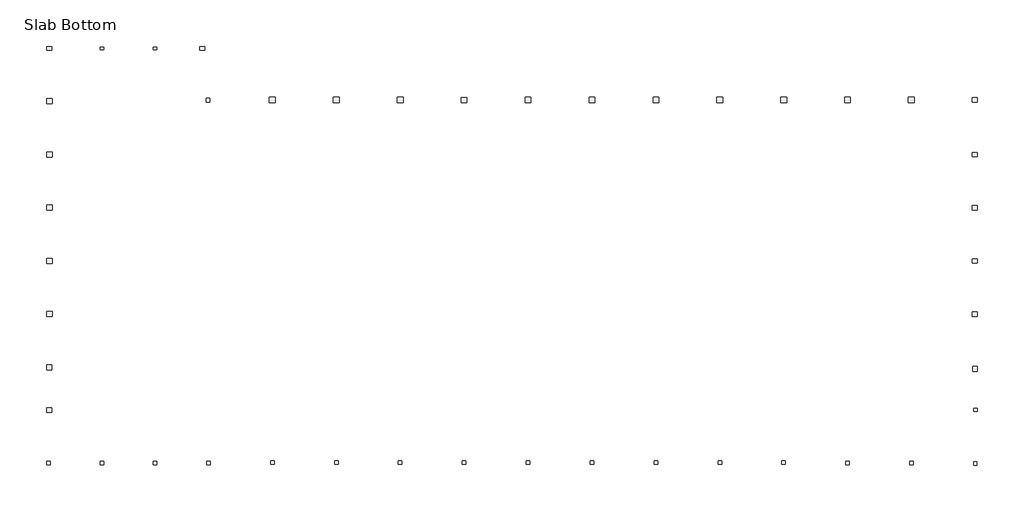
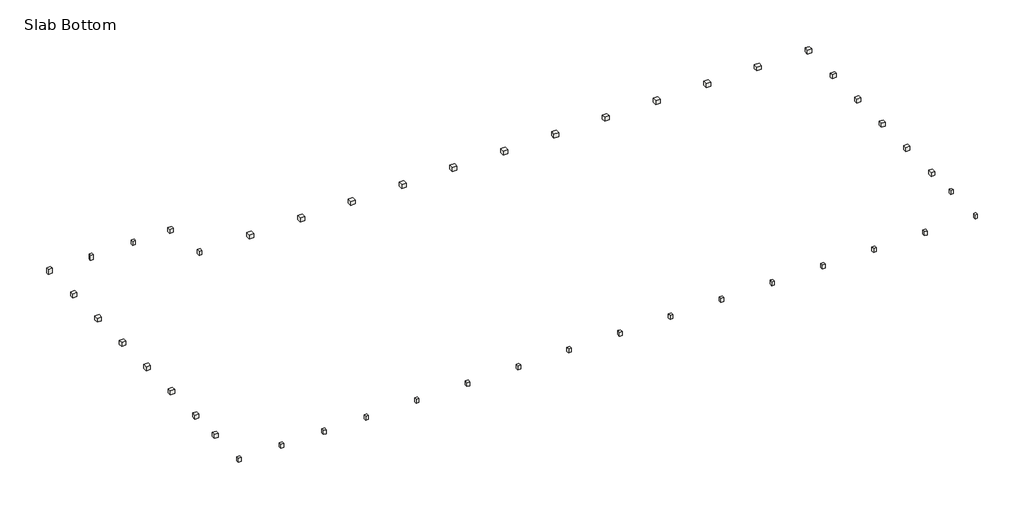
# One storey: 46 slabs.
"""IFC4 building model written with IfcOpenShell, lengths in millimetres."""

from ifc_helpers import new_model, si_unit, frame, origin, place, context, project, spatial, polyline, outline, extrude, faceted_brep, element, save

model = new_model("IFC4")

# Units and contexts
model_context = context("Model", 3, world=origin())
ifc_project = project(units=[si_unit("LENGTHUNIT", "METRE", prefix="MILLI")], contexts=[model_context])

# Site, building, storey
site = spatial("IfcSite", under=ifc_project)
building = spatial("IfcBuilding", under=site)
storey = spatial("IfcBuildingStorey", under=building, Name="Slab Bottom", Elevation=-152.4)

# Slabs
placement = place(None, origin())
element("IfcSlab", 1, ObjectType="Footing-Rectangular : P1", at=placement, inside=storey, context=model_context, shape_type="SweptSolid", body=[
    extrude(outline(polyline([(411310.2398264, -572441.1413841), (411665.8398264, -572441.1413841), (411665.8398264, -572745.9413841), (411310.2398264, -572745.9413841), (411310.2398264, -572441.1413841)])), frame((0.0, 0.0, -914.4), z_axis=(0.0, 0.0, 1.0), x_axis=(1.0, 0.0, 0.0)), (0.0, 0.0, 1.0), 609.6),
])
element("IfcSlab", 2, ObjectType="Footing-Rectangular : P11", at=placement, inside=storey, context=model_context, shape_type="SweptSolid", body=[
    extrude(outline(polyline([(411138.7898264, -549562.0913841), (411138.7898264, -549054.0913841), (411697.5898264, -549054.0913841), (411697.5898264, -549562.0913841), (411138.7898264, -549562.0913841)])), frame((0.0, 0.0, -914.4), z_axis=(0.0, 0.0, 1.0), x_axis=(1.0, 0.0, 0.0)), (0.0, 0.0, 1.0), 609.6),
])
element("IfcSlab", 3, ObjectType="Footing-Rectangular : P11A", at=placement, inside=storey, context=model_context, shape_type="SweptSolid", body=[
    extrude(outline(polyline([(411138.7898264, -561817.5913841), (411138.7898264, -561309.5913841), (411697.5898264, -561309.5913841), (411697.5898264, -561817.5913841), (411138.7898264, -561817.5913841)])), frame((0.0, 0.0, -914.4), z_axis=(0.0, 0.0, 1.0), x_axis=(1.0, 0.0, 0.0)), (0.0, 0.0, 1.0), 609.6),
])
element("IfcSlab", 4, ObjectType="Footing-Rectangular : P12", at=placement, inside=storey, context=model_context, shape_type="SweptSolid", body=[
    extrude(outline(polyline([(304649.2898264, -537331.9913841), (304649.2898264, -536773.1913841), (305258.8898264, -536773.1913841), (305258.8898264, -537331.9913841), (304649.2898264, -537331.9913841)])), frame((0.0, 0.0, -914.4), z_axis=(0.0, 0.0, 1.0), x_axis=(1.0, 0.0, 0.0)), (0.0, 0.0, 1.0), 609.6),
])
element("IfcSlab", 5, ObjectType="Footing-Rectangular : P12", at=placement, inside=storey, context=model_context, shape_type="SweptSolid", body=[
    extrude(outline(polyline([(304649.2898264, -543459.7413841), (304649.2898264, -542900.9413841), (305258.8898264, -542900.9413841), (305258.8898264, -543459.7413841), (304649.2898264, -543459.7413841)])), frame((0.0, 0.0, -914.4), z_axis=(0.0, 0.0, 1.0), x_axis=(1.0, 0.0, 0.0)), (0.0, 0.0, 1.0), 609.6),
])
element("IfcSlab", 6, ObjectType="Footing-Rectangular : P12", at=placement, inside=storey, context=model_context, shape_type="SweptSolid", body=[
    extrude(outline(polyline([(304649.2898264, -549587.4913841), (304649.2898264, -549028.6913841), (305258.8898264, -549028.6913841), (305258.8898264, -549587.4913841), (304649.2898264, -549587.4913841)])), frame((0.0, 0.0, -914.4), z_axis=(0.0, 0.0, 1.0), x_axis=(1.0, 0.0, 0.0)), (0.0, 0.0, 1.0), 609.6),
])
element("IfcSlab", 7, ObjectType="Footing-Rectangular : P12", at=placement, inside=storey, context=model_context, shape_type="SweptSolid", body=[
    extrude(outline(polyline([(304649.2898264, -555715.2413841), (304649.2898264, -555156.4413841), (305258.8898264, -555156.4413841), (305258.8898264, -555715.2413841), (304649.2898264, -555715.2413841)])), frame((0.0, 0.0, -914.4), z_axis=(0.0, 0.0, 1.0), x_axis=(1.0, 0.0, 0.0)), (0.0, 0.0, 1.0), 609.6),
])
element("IfcSlab", 8, ObjectType="Footing-Rectangular : P12", at=placement, inside=storey, context=model_context, shape_type="SweptSolid", body=[
    extrude(outline(polyline([(304649.2898264, -561842.9913841), (304649.2898264, -561284.1913841), (305258.8898264, -561284.1913841), (305258.8898264, -561842.9913841), (304649.2898264, -561842.9913841)])), frame((0.0, 0.0, -914.4), z_axis=(0.0, 0.0, 1.0), x_axis=(1.0, 0.0, 0.0)), (0.0, 0.0, 1.0), 609.6),
])
element("IfcSlab", 9, ObjectType="Footing-Rectangular : P12", at=placement, inside=storey, context=model_context, shape_type="SweptSolid", body=[
    extrude(outline(polyline([(304623.8898264, -567970.7413841), (304623.8898264, -567411.9413841), (305233.4898264, -567411.9413841), (305233.4898264, -567970.7413841), (304623.8898264, -567970.7413841)])), frame((0.0, 0.0, -914.4), z_axis=(0.0, 0.0, 1.0), x_axis=(1.0, 0.0, 0.0)), (0.0, 0.0, 1.0), 609.6),
])
element("IfcSlab", 10, ObjectType="Footing-Rectangular : P13", at=placement, inside=storey, context=model_context, shape_type="SweptSolid", body=[
    extrude(outline(polyline([(403777.974756, -536594.2315281), (404438.374756, -536594.2315281), (404438.374756, -537203.8315281), (403777.974756, -537203.8315281), (403777.974756, -536594.2315281)])), frame((0.0, 0.0, -914.4), z_axis=(0.0, 0.0, 1.0), x_axis=(1.0, 0.0, 0.0)), (0.0, 0.0, 1.0), 609.6),
])
element("IfcSlab", 11, ObjectType="Footing-Rectangular : P13", at=placement, inside=storey, context=model_context, shape_type="SweptSolid", body=[
    extrude(outline(polyline([(396451.2398264, -536601.7413358), (397111.6398264, -536601.7413358), (397111.6398264, -537211.3413358), (396451.2398264, -537211.3413358), (396451.2398264, -536601.7413358)])), frame((0.0, 0.0, -914.4), z_axis=(0.0, 0.0, 1.0), x_axis=(1.0, 0.0, 0.0)), (0.0, 0.0, 1.0), 609.6),
])
element("IfcSlab", 12, ObjectType="Footing-Rectangular : P13", at=placement, inside=storey, context=model_context, shape_type="SweptSolid", body=[
    extrude(outline(polyline([(389097.9398264, -536601.7413358), (389758.3398264, -536601.7413358), (389758.3398264, -537211.3413358), (389097.9398264, -537211.3413358), (389097.9398264, -536601.7413358)])), frame((0.0, 0.0, -914.4), z_axis=(0.0, 0.0, 1.0), x_axis=(1.0, 0.0, 0.0)), (0.0, 0.0, 1.0), 609.6),
])
element("IfcSlab", 13, ObjectType="Footing-Rectangular : P13", at=placement, inside=storey, context=model_context, shape_type="SweptSolid", body=[
    extrude(outline(polyline([(381744.6398264, -536601.7413358), (382405.0398264, -536601.7413358), (382405.0398264, -537211.3413358), (381744.6398264, -537211.3413358), (381744.6398264, -536601.7413358)])), frame((0.0, 0.0, -914.4), z_axis=(0.0, 0.0, 1.0), x_axis=(1.0, 0.0, 0.0)), (0.0, 0.0, 1.0), 609.6),
])
element("IfcSlab", 14, ObjectType="Footing-Rectangular : P13", at=placement, inside=storey, context=model_context, shape_type="SweptSolid", body=[
    extrude(outline(polyline([(374391.3398264, -536601.7413358), (375051.7398264, -536601.7413358), (375051.7398264, -537211.3413358), (374391.3398264, -537211.3413358), (374391.3398264, -536601.7413358)])), frame((0.0, 0.0, -914.4), z_axis=(0.0, 0.0, 1.0), x_axis=(1.0, 0.0, 0.0)), (0.0, 0.0, 1.0), 609.6),
])
element("IfcSlab", 15, ObjectType="Footing-Rectangular : P13", at=placement, inside=storey, context=model_context, shape_type="SweptSolid", body=[
    extrude(outline(polyline([(367038.0398264, -536601.7413358), (367698.4398264, -536601.7413358), (367698.4398264, -537211.3413358), (367038.0398264, -537211.3413358), (367038.0398264, -536601.7413358)])), frame((0.0, 0.0, -914.4), z_axis=(0.0, 0.0, 1.0), x_axis=(1.0, 0.0, 0.0)), (0.0, 0.0, 1.0), 609.6),
])
element("IfcSlab", 16, ObjectType="Footing-Rectangular : P13", at=placement, inside=storey, context=model_context, shape_type="SweptSolid", body=[
    extrude(outline(polyline([(359684.7398264, -536601.7413358), (360345.1398264, -536601.7413358), (360345.1398264, -537211.3413358), (359684.7398264, -537211.3413358), (359684.7398264, -536601.7413358)])), frame((0.0, 0.0, -914.4), z_axis=(0.0, 0.0, 1.0), x_axis=(1.0, 0.0, 0.0)), (0.0, 0.0, 1.0), 609.6),
])
element("IfcSlab", 17, ObjectType="Footing-Rectangular : P13", at=placement, inside=storey, context=model_context, shape_type="SweptSolid", body=[
    extrude(outline(polyline([(352331.4398264, -536614.4413358), (352991.8398264, -536614.4413358), (352991.8398264, -537224.0413358), (352331.4398264, -537224.0413358), (352331.4398264, -536614.4413358)])), frame((0.0, 0.0, -914.4), z_axis=(0.0, 0.0, 1.0), x_axis=(1.0, 0.0, 0.0)), (0.0, 0.0, 1.0), 609.6),
])
element("IfcSlab", 18, ObjectType="Footing-Rectangular : P13", at=placement, inside=storey, context=model_context, shape_type="SweptSolid", body=[
    extrude(outline(polyline([(344978.1398264, -536601.7413358), (345638.5398264, -536601.7413358), (345638.5398264, -537211.3413358), (344978.1398264, -537211.3413358), (344978.1398264, -536601.7413358)])), frame((0.0, 0.0, -914.4), z_axis=(0.0, 0.0, 1.0), x_axis=(1.0, 0.0, 0.0)), (0.0, 0.0, 1.0), 609.6),
])
element("IfcSlab", 19, ObjectType="Footing-Rectangular : P13", at=placement, inside=storey, context=model_context, shape_type="SweptSolid", body=[
    extrude(outline(polyline([(337624.8398264, -536601.7413358), (338285.2398264, -536601.7413358), (338285.2398264, -537211.3413358), (337624.8398264, -537211.3413358), (337624.8398264, -536601.7413358)])), frame((0.0, 0.0, -914.4), z_axis=(0.0, 0.0, 1.0), x_axis=(1.0, 0.0, 0.0)), (0.0, 0.0, 1.0), 609.6),
])
element("IfcSlab", 20, ObjectType="Footing-Rectangular : P13", at=placement, inside=storey, context=model_context, shape_type="SweptSolid", body=[
    extrude(outline(polyline([(330271.5398264, -536601.7413358), (330931.9398264, -536601.7413358), (330931.9398264, -537211.3413358), (330271.5398264, -537211.3413358), (330271.5398264, -536601.7413358)])), frame((0.0, 0.0, -914.4), z_axis=(0.0, 0.0, 1.0), x_axis=(1.0, 0.0, 0.0)), (0.0, 0.0, 1.0), 609.6),
])
element("IfcSlab", 21, ObjectType="Footing-Rectangular : P13A", at=placement, inside=storey, context=model_context, shape_type="SweptSolid", body=[
    extrude(outline(polyline([(411107.0397781, -536620.7913358), (411716.6397781, -536620.7913358), (411716.6397781, -537179.5913358), (411107.0397781, -537179.5913358), (411107.0397781, -536620.7913358)])), frame((0.0, 0.0, -914.4), z_axis=(0.0, 0.0, 1.0), x_axis=(1.0, 0.0, 0.0)), (0.0, 0.0, 1.0), 609.6),
])
element("IfcSlab", 22, ObjectType="Footing-Rectangular : P14", at=placement, inside=storey, context=model_context, shape_type="Brep", body=[
    faceted_brep([(304649.2898264, -572339.5413841, -304.8), (304649.2898264, -572847.5413841, -304.8), (305208.0898264, -572847.5413841, -304.8), (305208.0898264, -572810.8391729, -304.8), (305208.0898264, -572404.4391729, -304.8), (305208.0898264, -572339.5413841, -304.8), (304649.2898264, -572339.5413841, -914.4), (304649.2898264, -572847.5413841, -914.4), (305208.0898264, -572847.5413841, -914.4), (305208.0898264, -572339.5413841, -914.4)], [[[0, 1, 2, 3, 4, 5]], [[1, 0, 6, 7]], [[2, 1, 7, 8]], [[5, 4, 3, 2, 8, 9]], [[0, 5, 9, 6]], [[7, 6, 9, 8]]]),
])
element("IfcSlab", 23, ObjectType="Footing-Rectangular : P2", at=placement, inside=storey, context=model_context, shape_type="SweptSolid", body=[
    extrude(outline(polyline([(322797.5898264, -530747.0413841), (322797.5898264, -531153.4413841), (322238.7898264, -531153.4413841), (322238.7898264, -530747.0413841), (322797.5898264, -530747.0413841)])), frame((0.0, 0.0, -914.4), z_axis=(0.0, 0.0, 1.0), x_axis=(1.0, 0.0, 0.0)), (0.0, 0.0, 1.0), 609.6),
])
element("IfcSlab", 24, ObjectType="Footing-Rectangular : P3", at=placement, inside=storey, context=model_context, shape_type="SweptSolid", body=[
    extrude(outline(polyline([(411310.2398264, -578543.4913841), (411615.0398264, -578543.4913841), (411615.0398264, -578949.8913841), (411310.2398264, -578949.8913841), (411310.2398264, -578543.4913841)])), frame((0.0, 0.0, -914.4), z_axis=(0.0, 0.0, 1.0), x_axis=(1.0, 0.0, 0.0)), (0.0, 0.0, 1.0), 609.6),
])
element("IfcSlab", 25, ObjectType="Footing-Rectangular : P4", at=placement, inside=storey, context=model_context, shape_type="SweptSolid", body=[
    extrude(outline(polyline([(310789.7398264, -531108.9913841), (310789.7398264, -530804.1913841), (311196.1398264, -530804.1913841), (311196.1398264, -531108.9913841), (310789.7398264, -531108.9913841)])), frame((0.0, 0.0, -1066.8), z_axis=(0.0, 0.0, 1.0), x_axis=(1.0, 0.0, 0.0)), (0.0, 0.0, 1.0), 762.0),
])
element("IfcSlab", 26, ObjectType="Footing-Rectangular : P4", at=placement, inside=storey, context=model_context, shape_type="SweptSolid", body=[
    extrude(outline(polyline([(317323.8898264, -531108.9913841), (316917.4898264, -531108.9913841), (316917.4898264, -530804.1913841), (317323.8898264, -530804.1913841), (317323.8898264, -531108.9913841)])), frame((0.0, 0.0, -914.4), z_axis=(0.0, 0.0, 1.0), x_axis=(1.0, 0.0, 0.0)), (0.0, 0.0, 1.0), 609.6),
])
element("IfcSlab", 27, ObjectType="Footing-Rectangular : P5", at=placement, inside=storey, context=model_context, shape_type="SweptSolid", body=[
    extrude(outline(polyline([(311196.1398264, -578892.7413841), (310789.7398264, -578892.7413841), (310789.7398264, -578486.3413841), (311196.1398264, -578486.3413841), (311196.1398264, -578892.7413841)])), frame((0.0, 0.0, -914.4), z_axis=(0.0, 0.0, 1.0), x_axis=(1.0, 0.0, 0.0)), (0.0, 0.0, 1.0), 609.6),
])
element("IfcSlab", 28, ObjectType="Footing-Rectangular : P5", at=placement, inside=storey, context=model_context, shape_type="SweptSolid", body=[
    extrude(outline(polyline([(317327.0648264, -578937.1913841), (316920.6648264, -578937.1913841), (316920.6648264, -578530.7913841), (317327.0648264, -578530.7913841), (317327.0648264, -578937.1913841)])), frame((0.0, 0.0, -914.4), z_axis=(0.0, 0.0, 1.0), x_axis=(1.0, 0.0, 0.0)), (0.0, 0.0, 1.0), 609.6),
])
element("IfcSlab", 29, ObjectType="Footing-Rectangular : P5", at=placement, inside=storey, context=model_context, shape_type="SweptSolid", body=[
    extrude(outline(polyline([(330398.5398264, -578448.2413841), (330804.9398264, -578448.2413841), (330804.9398264, -578854.6413841), (330398.5398264, -578854.6413841), (330398.5398264, -578448.2413841)])), frame((0.0, 0.0, -914.4), z_axis=(0.0, 0.0, 1.0), x_axis=(1.0, 0.0, 0.0)), (0.0, 0.0, 1.0), 609.6),
])
element("IfcSlab", 30, ObjectType="Footing-Rectangular : P5", at=placement, inside=storey, context=model_context, shape_type="SweptSolid", body=[
    extrude(outline(polyline([(337751.8398264, -578448.2413841), (338158.2398264, -578448.2413841), (338158.2398264, -578854.6413841), (337751.8398264, -578854.6413841), (337751.8398264, -578448.2413841)])), frame((0.0, 0.0, -914.4), z_axis=(0.0, 0.0, 1.0), x_axis=(1.0, 0.0, 0.0)), (0.0, 0.0, 1.0), 609.6),
])
element("IfcSlab", 31, ObjectType="Footing-Rectangular : P5", at=placement, inside=storey, context=model_context, shape_type="SweptSolid", body=[
    extrude(outline(polyline([(345105.1398264, -578448.2413841), (345511.5398264, -578448.2413841), (345511.5398264, -578854.6413841), (345105.1398264, -578854.6413841), (345105.1398264, -578448.2413841)])), frame((0.0, 0.0, -914.4), z_axis=(0.0, 0.0, 1.0), x_axis=(1.0, 0.0, 0.0)), (0.0, 0.0, 1.0), 609.6),
])
element("IfcSlab", 32, ObjectType="Footing-Rectangular : P5", at=placement, inside=storey, context=model_context, shape_type="SweptSolid", body=[
    extrude(outline(polyline([(352458.4398264, -578448.2413841), (352864.8398264, -578448.2413841), (352864.8398264, -578854.6413841), (352458.4398264, -578854.6413841), (352458.4398264, -578448.2413841)])), frame((0.0, 0.0, -914.4), z_axis=(0.0, 0.0, 1.0), x_axis=(1.0, 0.0, 0.0)), (0.0, 0.0, 1.0), 609.6),
])
element("IfcSlab", 33, ObjectType="Footing-Rectangular : P5", at=placement, inside=storey, context=model_context, shape_type="SweptSolid", body=[
    extrude(outline(polyline([(359811.7398264, -578448.2413841), (360218.1398264, -578448.2413841), (360218.1398264, -578854.6413841), (359811.7398264, -578854.6413841), (359811.7398264, -578448.2413841)])), frame((0.0, 0.0, -914.4), z_axis=(0.0, 0.0, 1.0), x_axis=(1.0, 0.0, 0.0)), (0.0, 0.0, 1.0), 609.6),
])
element("IfcSlab", 34, ObjectType="Footing-Rectangular : P5", at=placement, inside=storey, context=model_context, shape_type="SweptSolid", body=[
    extrude(outline(polyline([(367165.0398264, -578448.2413841), (367571.4398264, -578448.2413841), (367571.4398264, -578854.6413841), (367165.0398264, -578854.6413841), (367165.0398264, -578448.2413841)])), frame((0.0, 0.0, -914.4), z_axis=(0.0, 0.0, 1.0), x_axis=(1.0, 0.0, 0.0)), (0.0, 0.0, 1.0), 609.6),
])
element("IfcSlab", 35, ObjectType="Footing-Rectangular : P5", at=placement, inside=storey, context=model_context, shape_type="SweptSolid", body=[
    extrude(outline(polyline([(374518.3398264, -578448.2413841), (374924.7398264, -578448.2413841), (374924.7398264, -578854.6413841), (374518.3398264, -578854.6413841), (374518.3398264, -578448.2413841)])), frame((0.0, 0.0, -914.4), z_axis=(0.0, 0.0, 1.0), x_axis=(1.0, 0.0, 0.0)), (0.0, 0.0, 1.0), 609.6),
])
element("IfcSlab", 36, ObjectType="Footing-Rectangular : P5", at=placement, inside=storey, context=model_context, shape_type="SweptSolid", body=[
    extrude(outline(polyline([(381871.6398264, -578448.2413841), (382278.0398264, -578448.2413841), (382278.0398264, -578854.6413841), (381871.6398264, -578854.6413841), (381871.6398264, -578448.2413841)])), frame((0.0, 0.0, -914.4), z_axis=(0.0, 0.0, 1.0), x_axis=(1.0, 0.0, 0.0)), (0.0, 0.0, 1.0), 609.6),
])
element("IfcSlab", 37, ObjectType="Footing-Rectangular : P5", at=placement, inside=storey, context=model_context, shape_type="SweptSolid", body=[
    extrude(outline(polyline([(389224.9398264, -578448.2413841), (389631.3398264, -578448.2413841), (389631.3398264, -578854.6413841), (389224.9398264, -578854.6413841), (389224.9398264, -578448.2413841)])), frame((0.0, 0.0, -914.4), z_axis=(0.0, 0.0, 1.0), x_axis=(1.0, 0.0, 0.0)), (0.0, 0.0, 1.0), 609.6),
])
element("IfcSlab", 38, ObjectType="Footing-Rectangular : P5", at=placement, inside=storey, context=model_context, shape_type="SweptSolid", body=[
    extrude(outline(polyline([(403931.5398264, -578530.7913841), (404337.9398264, -578530.7913841), (404337.9398264, -578937.1913841), (403931.5398264, -578937.1913841), (403931.5398264, -578530.7913841)])), frame((0.0, 0.0, -914.4), z_axis=(0.0, 0.0, 1.0), x_axis=(1.0, 0.0, 0.0)), (0.0, 0.0, 1.0), 609.6),
])
element("IfcSlab", 39, ObjectType="Footing-Rectangular : P5A", at=placement, inside=storey, context=model_context, shape_type="SweptSolid", body=[
    extrude(outline(polyline([(396578.2398264, -578530.7913841), (396984.6398264, -578530.7913841), (396984.6398264, -578937.1913841), (396578.2398264, -578937.1913841), (396578.2398264, -578530.7913841)])), frame((0.0, 0.0, -914.4), z_axis=(0.0, 0.0, 1.0), x_axis=(1.0, 0.0, 0.0)), (0.0, 0.0, 1.0), 609.6),
])
element("IfcSlab", 40, ObjectType="Footing-Rectangular : P5B", at=placement, inside=storey, context=model_context, shape_type="SweptSolid", body=[
    extrude(outline(polyline([(323064.2898264, -578899.0913841), (323064.2898264, -578492.6913841), (323470.6898264, -578492.6913841), (323470.6898264, -578899.0913841), (323064.2898264, -578899.0913841)])), frame((0.0, 0.0, -914.4), z_axis=(0.0, 0.0, 1.0), x_axis=(1.0, 0.0, 0.0)), (0.0, 0.0, 1.0), 609.6),
])
element("IfcSlab", 41, ObjectType="Footing-Rectangular : P5C", at=placement, inside=storey, context=model_context, shape_type="SweptSolid", body=[
    extrude(outline(polyline([(304642.9398264, -578899.0913841), (304642.9398264, -578492.6913841), (305049.3398264, -578492.6913841), (305049.3398264, -578899.0913841), (304642.9398264, -578899.0913841)])), frame((0.0, 0.0, -914.4), z_axis=(0.0, 0.0, 1.0), x_axis=(1.0, 0.0, 0.0)), (0.0, 0.0, 1.0), 609.6),
])
element("IfcSlab", 42, ObjectType="Footing-Rectangular : P6", at=placement, inside=storey, context=model_context, shape_type="SweptSolid", body=[
    extrude(outline(polyline([(323019.8398264, -536722.3913841), (323426.2398264, -536722.3913841), (323426.2398264, -537179.5913841), (323019.8398264, -537179.5913841), (323019.8398264, -536722.3913841)])), frame((0.0, 0.0, -914.4), z_axis=(0.0, 0.0, 1.0), x_axis=(1.0, 0.0, 0.0)), (0.0, 0.0, 1.0), 609.6),
])
element("IfcSlab", 43, ObjectType="Footing-Rectangular : P6A", at=placement, inside=storey, context=model_context, shape_type="SweptSolid", body=[
    extrude(outline(polyline([(304655.6398264, -530747.0413841), (305214.4398264, -530747.0413841), (305214.4398264, -531153.4413841), (304655.6398264, -531153.4413841), (304655.6398264, -530747.0413841)])), frame((0.0, 0.0, -1066.8), z_axis=(0.0, 0.0, 1.0), x_axis=(1.0, 0.0, 0.0)), (0.0, 0.0, 1.0), 762.0),
])
element("IfcSlab", 44, ObjectType="Footing-Rectangular : P7", at=placement, inside=storey, context=model_context, shape_type="SweptSolid", body=[
    extrude(outline(polyline([(411157.8398264, -567577.0413841), (411665.8398264, -567577.0413841), (411665.8398264, -568135.8413841), (411157.8398264, -568135.8413841), (411157.8398264, -567577.0413841)])), frame((0.0, 0.0, -914.4), z_axis=(0.0, 0.0, 1.0), x_axis=(1.0, 0.0, 0.0)), (0.0, 0.0, 1.0), 609.6),
])
element("IfcSlab", 45, ObjectType="Footing-Rectangular : P8", at=placement, inside=storey, context=model_context, shape_type="SweptSolid", body=[
    extrude(outline(polyline([(411138.7898264, -555664.4413841), (411138.7898264, -555207.2413841), (411697.5898264, -555207.2413841), (411697.5898264, -555664.4413841), (411138.7898264, -555664.4413841)])), frame((0.0, 0.0, -914.4), z_axis=(0.0, 0.0, 1.0), x_axis=(1.0, 0.0, 0.0)), (0.0, 0.0, 1.0), 609.6),
])
element("IfcSlab", 46, ObjectType="Footing-Rectangular : P9", at=placement, inside=storey, context=model_context, shape_type="SweptSolid", body=[
    extrude(outline(polyline([(411107.0398264, -543408.9413841), (411107.0398264, -542951.7413841), (411716.6398264, -542951.7413841), (411716.6398264, -543408.9413841), (411107.0398264, -543408.9413841)])), frame((0.0, 0.0, -914.4), z_axis=(0.0, 0.0, 1.0), x_axis=(1.0, 0.0, 0.0)), (0.0, 0.0, 1.0), 609.6),
])

save(model, "model.ifc")

# Revit data of these elements
# Type "Footing-Rectangular : P1"
#   Type Mark = ""
#   Assembly Code = "A1010100"
#   Width = 1' - 2"
#   Length = 1' - 0"
#   Thickness = 2' - 6"
#   Structural Material [instance default] = CONCRETE FOOTING - SEE STRUCT DWGS.
# Type "Footing-Rectangular : P11"
#   Assembly Code = "A1010100"
#   Width = 1' - 8"
#   Length = 1' - 10"
#   Thickness = 2' - 6"
#   Structural Material [instance default] = CONCRETE FOOTING - SEE STRUCT DWGS.
# Type "Footing-Rectangular : P11A"
#   Assembly Code = "A1010100"
#   Width = 1' - 8"
#   Length = 1' - 10"
#   Thickness = 2' - 6"
#   Structural Material [instance default] = CONCRETE FOOTING - SEE STRUCT DWGS.
# Type "Footing-Rectangular : P12"
#   Assembly Code = "A1010100"
#   Width = 1' - 10"
#   Length = 2' - 0"
#   Thickness = 2' - 6"
#   Structural Material [instance default] = CONCRETE FOOTING - SEE STRUCT DWGS.
# Type "Footing-Rectangular : P13"
#   Assembly Code = "A1010100"
#   Width = 2' - 2"
#   Length = 2' - 0"
#   Thickness = 2' - 6"
#   Structural Material [instance default] = CONCRETE FOOTING - SEE STRUCT DWGS.
# Type "Footing-Rectangular : P13A"
#   Assembly Code = "A1010100"
#   Width = 2' - 0"
#   Length = 1' - 10"
#   Thickness = 2' - 6"
#   Structural Material [instance default] = CONCRETE FOOTING - SEE STRUCT DWGS.
# Type "Footing-Rectangular : P14"
#   Assembly Code = "A1010100"
#   Width = 1' - 8"
#   Length = 1' - 10"
#   Thickness = 2' - 6"
#   Structural Material [instance default] = CONCRETE FOOTING - SEE STRUCT DWGS.
# Type "Footing-Rectangular : P2"
#   Assembly Code = "A1010100"
#   Width = 1' - 4"
#   Length = 1' - 10"
#   Thickness = 2' - 6"
#   Structural Material [instance default] = CONCRETE FOOTING - SEE STRUCT DWGS.
# Type "Footing-Rectangular : P3"
#   Assembly Code = "A1010100"
#   Width = 1' - 0"
#   Length = 1' - 4"
#   Thickness = 2' - 6"
#   Structural Material [instance default] = CONCRETE FOOTING - SEE STRUCT DWGS.
# Type "Footing-Rectangular : P4"
#   Assembly Code = "A1010100"
#   Width = 1' - 4"
#   Length = 1' - 0"
#   Thickness = 2' - 6"
#   Structural Material [instance default] = CONCRETE FOOTING - SEE STRUCT DWGS.
# Type "Footing-Rectangular : P5"
#   Assembly Code = "A1010100"
#   Width = 1' - 4"
#   Length = 1' - 4"
#   Thickness = 2' - 6"
#   Structural Material [instance default] = CONCRETE FOOTING - SEE STRUCT DWGS.
# Type "Footing-Rectangular : P5A"
#   Assembly Code = "A1010100"
#   Width = 1' - 4"
#   Length = 1' - 4"
#   Thickness = 2' - 6"
#   Structural Material [instance default] = CONCRETE FOOTING - SEE STRUCT DWGS.
# Type "Footing-Rectangular : P5B"
#   Assembly Code = "A1010100"
#   Width = 1' - 4"
#   Length = 1' - 4"
#   Thickness = 2' - 6"
#   Structural Material [instance default] = CONCRETE FOOTING - SEE STRUCT DWGS.
# Type "Footing-Rectangular : P5C"
#   Assembly Code = "A1010100"
#   Width = 1' - 4"
#   Length = 1' - 4"
#   Thickness = 2' - 6"
#   Structural Material [instance default] = CONCRETE FOOTING - SEE STRUCT DWGS.
# Type "Footing-Rectangular : P6"
#   Assembly Code = "A1010100"
#   Width = 1' - 4"
#   Length = 1' - 6"
#   Thickness = 2' - 6"
#   Structural Material [instance default] = CONCRETE FOOTING - SEE STRUCT DWGS.
# Type "Footing-Rectangular : P6A"
#   Assembly Code = "A1010100"
#   Width = 1' - 4"
#   Length = 1' - 10"
#   Thickness = 2' - 6"
#   Structural Material [instance default] = CONCRETE FOOTING - SEE STRUCT DWGS.
# Type "Footing-Rectangular : P7"
#   Assembly Code = "A1010100"
#   Width = 1' - 8"
#   Length = 1' - 10"
#   Thickness = 2' - 6"
#   Structural Material [instance default] = CONCRETE FOOTING - SEE STRUCT DWGS.
# Type "Footing-Rectangular : P8"
#   Assembly Code = "A1010100"
#   Width = 1' - 6"
#   Length = 1' - 10"
#   Thickness = 2' - 6"
#   Structural Material [instance default] = CONCRETE FOOTING - SEE STRUCT DWGS.
# Type "Footing-Rectangular : P9"
#   Assembly Code = "A1010100"
#   Width = 1' - 6"
#   Length = 2' - 0"
#   Thickness = 2' - 6"
#   Structural Material [instance default] = CONCRETE FOOTING - SEE STRUCT DWGS.
# Element 1 (IfcSlab, "Footing-Rectangular : P1")
#   Comments = ""
#   Structural Material = CONCRETE PIER- SEE STRUCT DWGS.
#   Phase Created = New Construction
#   Materials on its faces: "CONCRETE PIER- SEE STRUCT DWGS.", "CONCRETE FOOTING - SEE STRUCT DWGS."
# Element 2 (IfcSlab, "Footing-Rectangular : P11")
#   Comments = ""
#   Structural Material = CONCRETE PIER- SEE STRUCT DWGS.
#   Phase Created = New Construction
#   Materials on its faces: "CONCRETE PIER- SEE STRUCT DWGS.", "CONCRETE FOOTING - SEE STRUCT DWGS."
# Element 3 (IfcSlab, "Footing-Rectangular : P11A")
#   Comments = ""
#   Structural Material = CONCRETE PIER- SEE STRUCT DWGS.
#   Phase Created = New Construction
#   Materials on its faces: "CONCRETE PIER- SEE STRUCT DWGS.", "CONCRETE FOOTING - SEE STRUCT DWGS."
# Elements 4, 5, 6, 7, 8, 9 (IfcSlab, "Footing-Rectangular : P12")
#   Comments = ""
#   Structural Material = CONCRETE PIER- SEE STRUCT DWGS.
#   Phase Created = New Construction
#   Materials on its faces: "CONCRETE PIER- SEE STRUCT DWGS.", "CONCRETE FOOTING - SEE STRUCT DWGS."
# Elements 10, 11, 12, 13, 14, 15, 16, 17, 18, 19, 20 (IfcSlab, "Footing-Rectangular : P13")
#   Comments = ""
#   Structural Material = CONCRETE PIER- SEE STRUCT DWGS.
#   Phase Created = New Construction
#   Materials on its faces: "CONCRETE PIER- SEE STRUCT DWGS.", "CONCRETE FOOTING - SEE STRUCT DWGS."
# Element 21 (IfcSlab, "Footing-Rectangular : P13A")
#   Comments = ""
#   Structural Material = CONCRETE PIER- SEE STRUCT DWGS.
#   Phase Created = New Construction
#   Materials on its faces: "CONCRETE PIER- SEE STRUCT DWGS.", "CONCRETE FOOTING - SEE STRUCT DWGS."
# Element 22 (IfcSlab, "Footing-Rectangular : P14")
#   Comments = ""
#   Structural Material = CONCRETE PIER- SEE STRUCT DWGS.
#   Phase Created = New Construction
#   Materials on its faces: "CONCRETE PIER- SEE STRUCT DWGS.", "CONCRETE FOOTING - SEE STRUCT DWGS."
# Element 23 (IfcSlab, "Footing-Rectangular : P2")
#   Comments = ""
#   Structural Material = CONCRETE PIER- SEE STRUCT DWGS.
#   Phase Created = New Construction
#   Materials on its faces: "CONCRETE PIER- SEE STRUCT DWGS.", "CONCRETE FOOTING - SEE STRUCT DWGS."
# Element 24 (IfcSlab, "Footing-Rectangular : P3")
#   Comments = ""
#   Structural Material = CONCRETE PIER- SEE STRUCT DWGS.
#   Phase Created = New Construction
#   Materials on its faces: "CONCRETE PIER- SEE STRUCT DWGS.", "CONCRETE FOOTING - SEE STRUCT DWGS."
# Element 25 (IfcSlab, "Footing-Rectangular : P4")
#   Comments = ""
#   Structural Material = CONCRETE PIER- SEE STRUCT DWGS.
#   Phase Created = New Construction
#   Materials on its faces: "CONCRETE PIER- SEE STRUCT DWGS."
# Element 26 (IfcSlab, "Footing-Rectangular : P4")
#   Comments = ""
#   Structural Material = CONCRETE PIER- SEE STRUCT DWGS.
#   Phase Created = New Construction
#   Materials on its faces: "CONCRETE PIER- SEE STRUCT DWGS.", "CONCRETE FOOTING - SEE STRUCT DWGS."
# Elements 27, 28, 29, 30, 31, 32, 33, 34, 35, 36, 37, 38 (IfcSlab, "Footing-Rectangular : P5")
#   Comments = ""
#   Structural Material = CONCRETE PIER- SEE STRUCT DWGS.
#   Phase Created = New Construction
#   Materials on its faces: "CONCRETE PIER- SEE STRUCT DWGS.", "CONCRETE FOOTING - SEE STRUCT DWGS."
# Element 39 (IfcSlab, "Footing-Rectangular : P5A")
#   Comments = ""
#   Structural Material = CONCRETE PIER- SEE STRUCT DWGS.
#   Phase Created = New Construction
#   Materials on its faces: "CONCRETE PIER- SEE STRUCT DWGS.", "CONCRETE FOOTING - SEE STRUCT DWGS."
# Element 40 (IfcSlab, "Footing-Rectangular : P5B")
#   Comments = ""
#   Structural Material = CONCRETE PIER- SEE STRUCT DWGS.
#   Phase Created = New Construction
#   Materials on its faces: "CONCRETE PIER- SEE STRUCT DWGS.", "CONCRETE FOOTING - SEE STRUCT DWGS."
# Element 41 (IfcSlab, "Footing-Rectangular : P5C")
#   Comments = ""
#   Structural Material = CONCRETE PIER- SEE STRUCT DWGS.
#   Phase Created = New Construction
#   Materials on its faces: "CONCRETE PIER- SEE STRUCT DWGS.", "CONCRETE FOOTING - SEE STRUCT DWGS."
# Element 42 (IfcSlab, "Footing-Rectangular : P6")
#   Comments = ""
#   Structural Material = CONCRETE PIER- SEE STRUCT DWGS.
#   Phase Created = New Construction
#   Materials on its faces: "CONCRETE PIER- SEE STRUCT DWGS.", "CONCRETE FOOTING - SEE STRUCT DWGS."
# Element 43 (IfcSlab, "Footing-Rectangular : P6A")
#   Comments = ""
#   Structural Material = CONCRETE PIER- SEE STRUCT DWGS.
#   Phase Created = New Construction
#   Materials on its faces: "CONCRETE PIER- SEE STRUCT DWGS."
# Element 44 (IfcSlab, "Footing-Rectangular : P7")
#   Comments = ""
#   Structural Material = CONCRETE PIER- SEE STRUCT DWGS.
#   Phase Created = New Construction
#   Materials on its faces: "CONCRETE PIER- SEE STRUCT DWGS.", "CONCRETE FOOTING - SEE STRUCT DWGS."
# Element 45 (IfcSlab, "Footing-Rectangular : P8")
#   Comments = ""
#   Structural Material = CONCRETE PIER- SEE STRUCT DWGS.
#   Phase Created = New Construction
#   Materials on its faces: "CONCRETE PIER- SEE STRUCT DWGS.", "CONCRETE FOOTING - SEE STRUCT DWGS."
# Element 46 (IfcSlab, "Footing-Rectangular : P9")
#   Comments = ""
#   Structural Material = CONCRETE PIER- SEE STRUCT DWGS.
#   Phase Created = New Construction
#   Materials on its faces: "CONCRETE PIER- SEE STRUCT DWGS.", "CONCRETE FOOTING - SEE STRUCT DWGS."
# Materials
#   "CONCRETE FOOTING - SEE STRUCT DWGS.": class "Concrete", colour RGB 192 192 192, transparency 0, Description = "Cast-in-place concrete", Cost = 0
#   "CONCRETE PIER- SEE STRUCT DWGS.": class "Concrete", colour RGB 192 192 192, transparency 0, Description = "Cast-in-place concrete", Cost = 0
